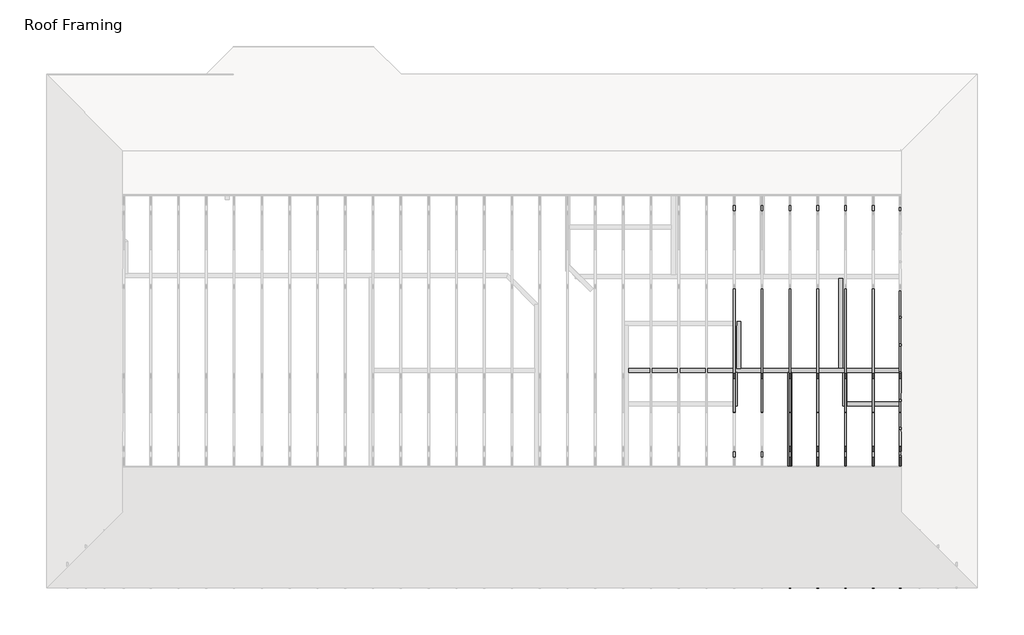
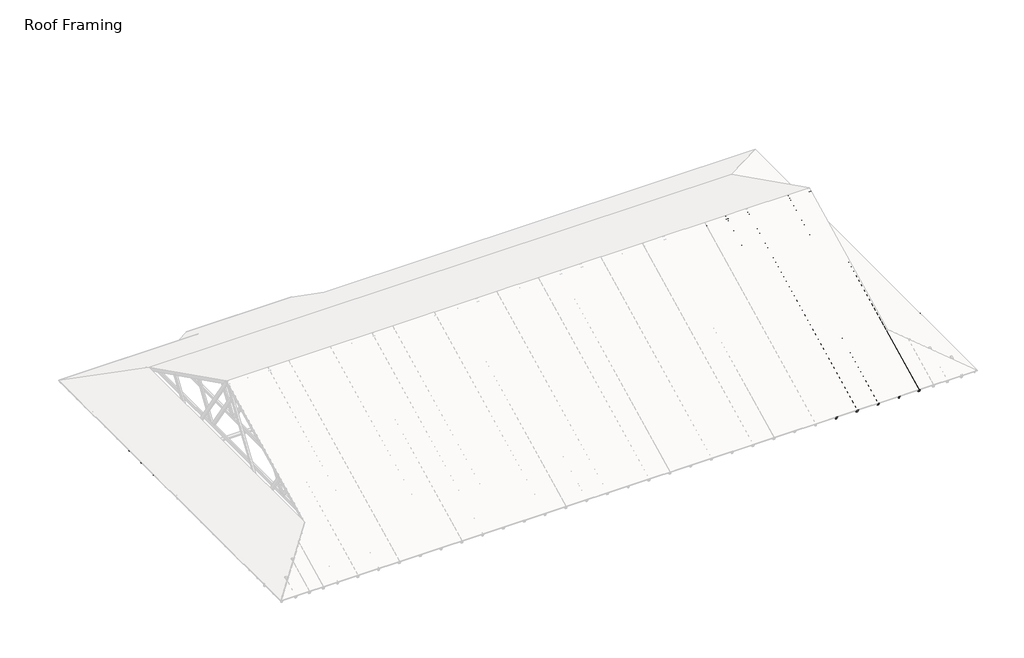
# One storey, part 4 of 7: 53 beams, 12 members.
"""IFC4 building model written with IfcOpenShell, lengths in millimetres."""

import ifcopenshell
import ifcopenshell.guid

model = None  # the IFC model being written
_history = None  # IfcOwnerHistory: only IFC2X3 demands one
_inside = {}  # id of a spatial element -> (the spatial element, [elements in it])
_under = {}  # id of a project, library or spatial element -> (it, [spatial elements below it])
_declared = {}  # id of a project -> (the project, [libraries it declares])
_typed = {}  # id of a type object -> (the type object, [elements of that type])
_made_of = {}  # id of a material, layer set ... -> (it, [elements and type objects made of it])


def new_model(schema):
    """Start an empty IFC model of exactly this schema.

    Asked for "IFC4X3", IfcOpenShell would pick the latest addendum, in which some entities
    have other attributes; the version numbers below select the first issue.
    IFC2X3 requires an IfcOwnerHistory on every rooted entity: one is made here for all.
    """
    global model, _history
    if schema == "IFC4X3":
        model = ifcopenshell.file(schema_version=(4, 3, 0, 0))
    else:
        model = ifcopenshell.file(schema=schema)
    _inside.clear()
    _under.clear()
    _declared.clear()
    _typed.clear()
    _made_of.clear()
    _history = None
    if model.schema == "IFC2X3":
        org = make("IfcOrganization", Name="unknown")
        user = make(
            "IfcPersonAndOrganization",
            ThePerson=make("IfcPerson", FamilyName="unknown"),
            TheOrganization=org,
        )
        app = make(
            "IfcApplication",
            ApplicationDeveloper=org,
            Version="unknown",
            ApplicationFullName="unknown",
            ApplicationIdentifier="unknown",
        )
        _history = make(
            "IfcOwnerHistory",
            OwningUser=user,
            OwningApplication=app,
            ChangeAction="ADDED",
            CreationDate=0,
        )
    return model


def make(cls, **values):
    """One entity of the class cls with the attributes given. An attribute that is None is left unset."""
    return model.create_entity(
        cls, **{name: value for name, value in values.items() if value is not None}
    )


def rooted(cls, **values):
    """An entity with a GlobalId (a new one), such as an element, a storey or a relation."""
    return make(cls, GlobalId=ifcopenshell.guid.new(), OwnerHistory=_history, **values)


def si_unit(unit_type, name, prefix=None):
    """IfcSIUnit, for example si_unit("LENGTHUNIT", "METRE", prefix="MILLI")."""
    return make("IfcSIUnit", UnitType=unit_type, Prefix=prefix, Name=name)


def assignment(units):
    """IfcUnitAssignment: the units of a project."""
    return None if units is None else make("IfcUnitAssignment", Units=units)


def point(xyz):
    """IfcCartesianPoint."""
    return None if xyz is None else make("IfcCartesianPoint", Coordinates=xyz)


def direction(xyz):
    """IfcDirection."""
    return None if xyz is None else make("IfcDirection", DirectionRatios=xyz)


def frame(location, z_axis=None, x_axis=None):
    """IfcAxis2Placement3D, a coordinate frame: its origin and axes. An axis left out is left unset."""
    return make(
        "IfcAxis2Placement3D",
        Location=point(location),
        Axis=direction(z_axis),
        RefDirection=direction(x_axis),
    )


def origin():
    """The frame at (0, 0, 0) with its axes left unset."""
    return frame((0.0, 0.0, 0.0))


def place(relative_to, where):
    """IfcLocalPlacement: puts the frame where relative to a parent placement (None: the world)."""
    return make(
        "IfcLocalPlacement", PlacementRelTo=relative_to, RelativePlacement=where
    )


def context(
    kind, dimensions, precision=None, world=None, true_north=None, identifier=None
):
    """IfcGeometricRepresentationContext, for example the 3D "Model" context."""
    return make(
        "IfcGeometricRepresentationContext",
        ContextIdentifier=identifier,
        ContextType=kind,
        CoordinateSpaceDimension=dimensions,
        Precision=precision,
        WorldCoordinateSystem=world,
        TrueNorth=true_north,
    )


def project(units=None, contexts=None):
    """IfcProject with its units and contexts."""
    return rooted(
        "IfcProject",
        Name="project",
        RepresentationContexts=contexts,
        UnitsInContext=assignment(units),
    )


def spatial(cls, under=None, at=None, **own):
    """A site, building, storey or space (cls), placed at a placement, below another one or the project."""
    s = rooted(cls, ObjectPlacement=at, **own)
    if under is not None:
        _under.setdefault(under.id(), (under, []))[1].append(s)
    return s


def polyline(points):
    """IfcPolyline through the points."""
    return make("IfcPolyline", Points=[point(p) for p in points])


def outline(outer, holes=None, kind="AREA"):
    """IfcArbitraryClosedProfileDef: a profile drawn as a closed curve; with holes, ...WithVoids."""
    if holes is None:
        return make("IfcArbitraryClosedProfileDef", ProfileType=kind, OuterCurve=outer)
    return make(
        "IfcArbitraryProfileDefWithVoids",
        ProfileType=kind,
        OuterCurve=outer,
        InnerCurves=holes,
    )


def extrude(swept, where, along, depth):
    """IfcExtrudedAreaSolid: the profile swept, set in the frame where, extruded along a direction by depth."""
    return make(
        "IfcExtrudedAreaSolid",
        SweptArea=swept,
        Position=where,
        ExtrudedDirection=direction(along),
        Depth=depth,
    )


def shape(context_of_items, identifier, shape_type, items):
    """IfcShapeRepresentation: the items that make up one representation, for example the "Body"."""
    return make(
        "IfcShapeRepresentation",
        ContextOfItems=context_of_items,
        RepresentationIdentifier=identifier,
        RepresentationType=shape_type,
        Items=items,
    )


def source(mapping_origin, context_of_items, identifier, shape_type, items):
    """IfcRepresentationMap: a shape defined once, which mapped items show again and again."""
    return make(
        "IfcRepresentationMap",
        MappingOrigin=mapping_origin,
        MappedRepresentation=shape(context_of_items, identifier, shape_type, items),
    )


def transform(
    local_origin,
    x_axis=None,
    y_axis=None,
    z_axis=None,
    scale=None,
    scale2=None,
    scale3=None,
    uniform=True,
):
    """IfcCartesianTransformationOperator3D, or its non-uniform kind. x_axis, y_axis, z_axis: its Axis1, 2, 3."""
    if uniform:
        return make(
            "IfcCartesianTransformationOperator3D",
            Axis1=direction(x_axis),
            Axis2=direction(y_axis),
            LocalOrigin=point(local_origin),
            Scale=scale,
            Axis3=direction(z_axis),
        )
    return make(
        "IfcCartesianTransformationOperator3DnonUniform",
        Axis1=direction(x_axis),
        Axis2=direction(y_axis),
        LocalOrigin=point(local_origin),
        Scale=scale,
        Axis3=direction(z_axis),
        Scale2=scale2,
        Scale3=scale3,
    )


def mapped(mapping_source, mapping_target):
    """IfcMappedItem: shows the shape of a source again, moved by a transform."""
    return make(
        "IfcMappedItem", MappingSource=mapping_source, MappingTarget=mapping_target
    )


def made_of(thing, what):
    """Note that an element or type object is made of a material, layer set ...; save() writes the relation."""
    if what is not None:
        _made_of.setdefault(what.id(), (what, []))[1].append(thing)
    return thing


def element(
    cls,
    number,
    at=None,
    inside=None,
    cuts=None,
    type_object=None,
    material=None,
    context=None,
    identifier="Body",
    shape_type=None,
    held_by="IfcProductDefinitionShape",
    body=None,
    shapes=None,
    **own,
):
    """One element of the class cls, such as IfcWall. Its Tag is "e" and its number.

    at: its placement. inside: the storey or other place that contains it. cuts: it is an
    opening in that element (IfcRelVoidsElement). A single representation is given by context,
    identifier, shape_type and body (its items); several are given by shapes. held_by: the class
    of the entity that holds the representations. save() writes the other relations.
    """
    e = rooted(cls, Tag="e%d" % number, ObjectPlacement=at, **own)
    if body is not None:
        shapes = [shape(context, identifier, shape_type, body)]
    if shapes is not None:
        e.Representation = make(held_by, Representations=shapes)
    if inside is not None:
        _inside.setdefault(inside.id(), (inside, []))[1].append(e)
    if cuts is not None:
        rooted(
            "IfcRelVoidsElement", RelatingBuildingElement=cuts, RelatedOpeningElement=e
        )
    if type_object is not None:
        _typed.setdefault(type_object.id(), (type_object, []))[1].append(e)
    return made_of(e, material)


def aggregate(whole, parts):
    """IfcRelAggregates: a whole, such as a stair, and the parts it consists of."""
    return rooted("IfcRelAggregates", RelatingObject=whole, RelatedObjects=parts)


def save(model, path):
    """Write the relations noted so far, then the file.

    IfcRelAggregates (storeys below a building ...), IfcRelContainedInSpatialStructure (elements
    in a storey), IfcRelDefinesByType, IfcRelAssociatesMaterial and IfcRelDeclares: one each for
    every whole, place, type object, material and project.
    """
    for whole, parts in _under.values():
        aggregate(whole, parts)
    for where, things in _inside.values():
        rooted(
            "IfcRelContainedInSpatialStructure",
            RelatedElements=things,
            RelatingStructure=where,
        )
    for kind, things in _typed.values():
        rooted("IfcRelDefinesByType", RelatedObjects=things, RelatingType=kind)
    for what, things in _made_of.values():
        rooted("IfcRelAssociatesMaterial", RelatedObjects=things, RelatingMaterial=what)
    for by, libraries in _declared.values():
        rooted("IfcRelDeclares", RelatingContext=by, RelatedDefinitions=libraries)
    model.write(path)


def dimension_lumber_c8f8d63a(model_context):
    return source(origin(), model_context, "Body", "SweptSolid", [
        extrude(outline(polyline([(5118.89375, 44.45), (5118.89375, -44.45), (-5118.89375, -44.45), (-5118.89375, 44.45), (5118.89375, 44.45)])), frame((0.0, 0.0, -19.05), z_axis=(0.0, 0.0, 1.0), x_axis=(1.0, 0.0, 0.0)), (0.0, 0.0, 1.0), 38.1),
    ])


def dimension_lumber_b8718559(model_context):
    return source(origin(), model_context, "Body", "SweptSolid", [
        extrude(outline(polyline([(987.425, 44.45), (987.425, -44.45), (-987.425, -44.45), (-987.425, 44.45), (987.425, 44.45)])), frame((0.0, 0.0, -19.05), z_axis=(0.0, 0.0, 1.0), x_axis=(1.0, 0.0, 0.0)), (0.0, 0.0, 1.0), 38.1),
    ])


def dimension_lumber_96205b60(model_context):
    return source(origin(), model_context, "Body", "SweptSolid", [
        extrude(outline(polyline([(3550.44375, 44.45), (3550.44375, -44.45), (-3550.44375, -44.45), (-3550.44375, 44.45), (3550.44375, 44.45)])), frame((0.0, 0.0, -19.05), z_axis=(0.0, 0.0, 1.0), x_axis=(1.0, 0.0, 0.0)), (0.0, 0.0, 1.0), 38.1),
    ])


def dimension_lumber_dd19c813(model_context):
    return source(origin(), model_context, "Body", "SweptSolid", [
        extrude(outline(polyline([(558.8, 44.45), (558.8, -44.45), (-469.9, -44.45), (-469.9, 44.45), (558.8, 44.45)])), frame((0.0, 0.0, -19.05), z_axis=(0.0, 0.0, 1.0), x_axis=(1.0, 0.0, 0.0)), (0.0, 0.0, 1.0), 38.1),
    ])


def dimension_lumber_d9c95be3(model_context):
    return source(origin(), model_context, "Body", "SweptSolid", [
        extrude(outline(polyline([(346.075, 44.45), (346.075, -44.45), (-384.175, -44.45), (-384.175, 44.45), (346.075, 44.45)])), frame((0.0, 0.0, -19.05), z_axis=(0.0, 0.0, 1.0), x_axis=(1.0, 0.0, 0.0)), (0.0, 0.0, 1.0), 38.1),
    ])


def dimension_lumber_c20748c8(model_context):
    return source(origin(), model_context, "Body", "SweptSolid", [
        extrude(outline(polyline([(1155.7, 44.45), (1155.7, -44.45), (-1155.7, -44.45), (-1155.7, 44.45), (1155.7, 44.45)])), frame((0.0, 0.0, -19.05), z_axis=(0.0, 0.0, 1.0), x_axis=(1.0, 0.0, 0.0)), (0.0, 0.0, 1.0), 38.1),
    ])


def dimension_lumber_348b767d(model_context):
    return source(origin(), model_context, "Body", "SweptSolid", [
        extrude(outline(polyline([(320.675, 44.45), (320.675, -44.45), (-409.575, -44.45), (-409.575, 44.45), (320.675, 44.45)])), frame((0.0, 0.0, -19.05), z_axis=(0.0, 0.0, 1.0), x_axis=(1.0, 0.0, 0.0)), (0.0, 0.0, 1.0), 38.1),
    ])


def dimension_lumber_22ea9708(model_context):
    return source(origin(), model_context, "Body", "SweptSolid", [
        extrude(outline(polyline([(2035.175, 44.45), (2035.175, -44.45), (-2035.175, -44.45), (-2035.175, 44.45), (2035.175, 44.45)])), frame((0.0, 0.0, -19.05), z_axis=(0.0, 0.0, 1.0), x_axis=(1.0, 0.0, 0.0)), (0.0, 0.0, 1.0), 38.1),
    ])


def dimension_lumber_74193215(model_context):
    return source(origin(), model_context, "Body", "SweptSolid", [
        extrude(outline(polyline([(409.575, 44.45), (409.575, -44.45), (-320.675, -44.45), (-320.675, 44.45), (409.575, 44.45)])), frame((0.0, 0.0, -19.05), z_axis=(0.0, 0.0, 1.0), x_axis=(1.0, 0.0, 0.0)), (0.0, 0.0, 1.0), 38.1),
    ])


def dimension_lumber_7189ff9c(model_context):
    return source(origin(), model_context, "Body", "SweptSolid", [
        extrude(outline(polyline([(1146.96875, 44.45), (1146.96875, -44.45), (-1164.43125, -44.45), (-1164.43125, 44.45), (1146.96875, 44.45)])), frame((0.0, 0.0, -19.05), z_axis=(0.0, 0.0, 1.0), x_axis=(1.0, 0.0, 0.0)), (0.0, 0.0, 1.0), 38.1),
    ])


def dimension_lumber_f425b765(model_context):
    return source(origin(), model_context, "Body", "SweptSolid", [
        extrude(outline(polyline([(292.0, 44.45), (292.0, -44.45), (-165.0, -44.45), (-165.0, 44.45), (292.0, 44.45)])), frame((0.0, 0.0, -19.05), z_axis=(0.0, 0.0, 1.0), x_axis=(1.0, 0.0, 0.0)), (0.0, 0.0, 1.0), 38.1),
    ])


def dimension_lumber_supporting_bottom_plate_e3733361(model_context):
    return source(origin(), model_context, "Body", "SweptSolid", [
        extrude(outline(polyline([(328.9051334, 44.45), (328.9051334, -44.45), (-328.9051334, -44.45), (-328.9051334, 44.45), (328.9051334, 44.45)])), frame((0.0, 0.0, -19.05), z_axis=(0.0, 0.0, 1.0), x_axis=(1.0, 0.0, 0.0)), (0.0, 0.0, 1.0), 38.1),
    ])


def dimension_lumber_supporting_bottom_plate_47a8c852(model_context):
    return source(origin(), model_context, "Body", "SweptSolid", [
        extrude(outline(polyline([(292.0, 44.45), (292.0, -44.45), (-203.1, -44.45), (-203.1, 44.45), (292.0, 44.45)])), frame((0.0, 0.0, -19.05), z_axis=(0.0, 0.0, 1.0), x_axis=(1.0, 0.0, 0.0)), (0.0, 0.0, 1.0), 38.1),
    ])


model = new_model("IFC4")

# Units and contexts
model_context = context("Model", 3, world=origin())
ifc_project = project(units=[si_unit("LENGTHUNIT", "METRE", prefix="MILLI")], contexts=[model_context])

# Site, building, storey
site = spatial("IfcSite", under=ifc_project)
building = spatial("IfcBuilding", under=site)
storey = spatial("IfcBuildingStorey", under=building, Name="Roof Framing", Elevation=2768.6)

# Beams
placement = place(None, origin())
element("IfcBeam", 1, ObjectType="Dimension Lumber : Roof Lumbers", at=placement, inside=storey, context=model_context, shape_type="SweptSolid", body=[
    extrude(outline(polyline([(0.0, -38.1), (0.0, 0.0), (1874.2721787, 0.0), (1874.2721787, -38.1), (0.0, -38.1)])), frame((13672.6274862, -3444.5040947, 2554.840297), z_axis=(0.44721359549993345, 0.0, 0.8944271909999282), x_axis=(-0.8944271909999282, 0.0, 0.44721359549993345)), (0.0, 0.0, 1.0), 88.9),
    extrude(outline(polyline([(2554.840297, 13672.6274862), (2558.1548743, 13674.2847749), (2653.4048743, 13674.2847749), (3472.5548743, 12035.9847749), (3393.040297, 11996.2274862), (2554.840297, 13672.6274862)])), frame((0.0, -3444.5040947, 0.0), z_axis=(0.0, 1.0, 0.0), x_axis=(0.0, 0.0, 1.0)), (0.0, 0.0, 1.0), 38.1),
    extrude(outline(polyline([(2554.840297, 13672.6274862), (2558.1548743, 13674.2847749), (2653.4048743, 13674.2847749), (3472.5548743, 12035.9847749), (3373.1616527, 12035.9847749), (2554.840297, 13672.6274862)])), frame((0.0, -3444.5040947, 0.0), z_axis=(0.0, 1.0, 0.0), x_axis=(0.0, 0.0, 1.0)), (0.0, 0.0, 1.0), 38.1),
])
element("IfcBeam", 2, ObjectType="Dimension Lumber : Roof Lumbers", at=placement, inside=storey, context=model_context, shape_type="SweptSolid", body=[
    extrude(outline(polyline([(0.0, -38.1), (0.0, 0.0), (1874.2721787, 0.0), (1874.2721787, -38.1), (0.0, -38.1)])), frame((13672.6274862, -2834.9040947, 2554.840297), z_axis=(0.44721359549993345, 0.0, 0.8944271909999282), x_axis=(-0.8944271909999282, 0.0, 0.44721359549993345)), (0.0, 0.0, 1.0), 88.9),
    extrude(outline(polyline([(2554.840297, 13672.6274862), (2558.1548743, 13674.2847749), (2653.4048743, 13674.2847749), (3472.5548743, 12035.9847749), (3393.040297, 11996.2274862), (2554.840297, 13672.6274862)])), frame((0.0, -2834.9040947, 0.0), z_axis=(0.0, 1.0, 0.0), x_axis=(0.0, 0.0, 1.0)), (0.0, 0.0, 1.0), 38.1),
    extrude(outline(polyline([(2554.840297, 13672.6274862), (2558.1548743, 13674.2847749), (2653.4048743, 13674.2847749), (3472.5548743, 12035.9847749), (3373.1616527, 12035.9847749), (2554.840297, 13672.6274862)])), frame((0.0, -2834.9040947, 0.0), z_axis=(0.0, 1.0, 0.0), x_axis=(0.0, 0.0, 1.0)), (0.0, 0.0, 1.0), 38.1),
])
element("IfcBeam", 3, ObjectType="Dimension Lumber : Roof Lumbers", at=placement, inside=storey, context=model_context, shape_type="SweptSolid", body=[
    extrude(outline(polyline([(0.0, -38.1), (0.0, 0.0), (1874.2721787, 0.0), (1874.2721787, -38.1), (0.0, -38.1)])), frame((13672.6274862, -2225.3040947, 2554.840297), z_axis=(0.44721359549993345, 0.0, 0.8944271909999282), x_axis=(-0.8944271909999282, 0.0, 0.44721359549993345)), (0.0, 0.0, 1.0), 88.9),
    extrude(outline(polyline([(2554.840297, 13672.6274862), (2558.1548743, 13674.2847749), (2653.4048743, 13674.2847749), (3472.5548743, 12035.9847749), (3393.040297, 11996.2274862), (2554.840297, 13672.6274862)])), frame((0.0, -2225.3040947, 0.0), z_axis=(0.0, 1.0, 0.0), x_axis=(0.0, 0.0, 1.0)), (0.0, 0.0, 1.0), 38.1),
    extrude(outline(polyline([(2554.840297, 13672.6274862), (2558.1548743, 13674.2847749), (2653.4048743, 13674.2847749), (3472.5548743, 12035.9847749), (3373.1616527, 12035.9847749), (2554.840297, 13672.6274862)])), frame((0.0, -2225.3040947, 0.0), z_axis=(0.0, 1.0, 0.0), x_axis=(0.0, 0.0, 1.0)), (0.0, 0.0, 1.0), 38.1),
])
element("IfcBeam", 4, ObjectType="Dimension Lumber : Roof Lumbers", at=placement, inside=storey, context=model_context, shape_type="SweptSolid", body=[
    extrude(outline(polyline([(0.0, -38.1), (0.0, 0.0), (1874.2721787, 0.0), (1874.2721787, -38.1), (0.0, -38.1)])), frame((13672.6274862, -1006.1040947, 2554.840297), z_axis=(0.44721359549993367, 0.0, 0.8944271909999281), x_axis=(-0.8944271909999281, 0.0, 0.44721359549993367)), (0.0, 0.0, 1.0), 88.9),
    extrude(outline(polyline([(2554.840297, 13672.6274862), (2558.1548743, 13674.2847749), (2653.4048743, 13674.2847749), (3472.5548743, 12035.9847749), (3393.040297, 11996.2274862), (2554.840297, 13672.6274862)])), frame((0.0, -1006.1040947, 0.0), z_axis=(0.0, 1.0, 0.0), x_axis=(0.0, 0.0, 1.0)), (0.0, 0.0, 1.0), 38.1),
    extrude(outline(polyline([(2554.840297, 13672.6274862), (2558.1548743, 13674.2847749), (2653.4048743, 13674.2847749), (3472.5548743, 12035.9847749), (3373.1616527, 12035.9847749), (2554.840297, 13672.6274862)])), frame((0.0, -1006.1040947, 0.0), z_axis=(0.0, 1.0, 0.0), x_axis=(0.0, 0.0, 1.0)), (0.0, 0.0, 1.0), 38.1),
])
element("IfcBeam", 5, ObjectType="Dimension Lumber : Roof Lumbers", at=placement, inside=storey, context=model_context, shape_type="SweptSolid", body=[
    extrude(outline(polyline([(0.0, -38.1), (0.0, 0.0), (1874.2721787, 0.0), (1874.2721787, -38.1), (0.0, -38.1)])), frame((13672.6274862, -396.5040947, 2554.840297), z_axis=(0.44721359549993345, 0.0, 0.8944271909999282), x_axis=(-0.8944271909999282, 0.0, 0.44721359549993345)), (0.0, 0.0, 1.0), 88.9),
    extrude(outline(polyline([(2554.840297, 13672.6274862), (2558.1548743, 13674.2847749), (2653.4048743, 13674.2847749), (3472.5548743, 12035.9847749), (3393.040297, 11996.2274862), (2554.840297, 13672.6274862)])), frame((0.0, -396.5040947, 0.0), z_axis=(0.0, 1.0, 0.0), x_axis=(0.0, 0.0, 1.0)), (0.0, 0.0, 1.0), 38.1),
    extrude(outline(polyline([(2554.840297, 13672.6274862), (2558.1548743, 13674.2847749), (2653.4048743, 13674.2847749), (3472.5548743, 12035.9847749), (3373.1616527, 12035.9847749), (2554.840297, 13672.6274862)])), frame((0.0, -396.5040947, 0.0), z_axis=(0.0, 1.0, 0.0), x_axis=(0.0, 0.0, 1.0)), (0.0, 0.0, 1.0), 38.1),
])
element("IfcBeam", 6, ObjectType="Dimension Lumber : Roof Lumbers", at=placement, inside=storey, context=model_context, shape_type="SweptSolid", body=[
    extrude(outline(polyline([(12035.9847749, -3406.4040947), (13244.0722749, -3406.4040947), (13244.0722749, -3444.5040947), (12035.9847749, -3444.5040947), (12035.9847749, -3406.4040947)])), frame((0.0, 0.0, 2768.6), z_axis=(0.0, 0.0, 1.0), x_axis=(1.0, 0.0, 0.0)), (0.0, 0.0, 1.0), 88.9),
    extrude(outline(polyline([(2768.6, 12035.9847749), (2768.6, 13244.0722749), (2769.1179027, 13244.0722749), (2857.5, 13067.3080803), (2857.5, 12035.9847749), (2768.6, 12035.9847749)])), frame((0.0, -3444.5040947, 0.0), z_axis=(0.0, 1.0, 0.0), x_axis=(0.0, 0.0, 1.0)), (0.0, 0.0, 1.0), 38.1),
])
element("IfcBeam", 7, ObjectType="Dimension Lumber : Roof Lumbers", at=placement, inside=storey, context=model_context, shape_type="SweptSolid", body=[
    extrude(outline(polyline([(12035.9847749, -2796.8040947), (13244.0722749, -2796.8040947), (13244.0722749, -2834.9040947), (12035.9847749, -2834.9040947), (12035.9847749, -2796.8040947)])), frame((0.0, 0.0, 2768.6), z_axis=(0.0, 0.0, 1.0), x_axis=(1.0, 0.0, 0.0)), (0.0, 0.0, 1.0), 88.9),
    extrude(outline(polyline([(2768.6, 12035.9847749), (2768.6, 13244.0722749), (2769.1179027, 13244.0722749), (2857.5, 13067.3080803), (2857.5, 12035.9847749), (2768.6, 12035.9847749)])), frame((0.0, -2834.9040947, 0.0), z_axis=(0.0, 1.0, 0.0), x_axis=(0.0, 0.0, 1.0)), (0.0, 0.0, 1.0), 38.1),
])
element("IfcBeam", 8, ObjectType="Dimension Lumber : Roof Lumbers", at=placement, inside=storey, context=model_context, shape_type="SweptSolid", body=[
    extrude(outline(polyline([(12035.9847749, -2187.2040947), (13244.0722749, -2187.2040947), (13244.0722749, -2225.3040947), (12035.9847749, -2225.3040947), (12035.9847749, -2187.2040947)])), frame((0.0, 0.0, 2768.6), z_axis=(0.0, 0.0, 1.0), x_axis=(1.0, 0.0, 0.0)), (0.0, 0.0, 1.0), 88.9),
    extrude(outline(polyline([(2768.6, 12035.9847749), (2768.6, 13244.0722749), (2769.1179027, 13244.0722749), (2857.5, 13067.3080803), (2857.5, 12035.9847749), (2768.6, 12035.9847749)])), frame((0.0, -2225.3040947, 0.0), z_axis=(0.0, 1.0, 0.0), x_axis=(0.0, 0.0, 1.0)), (0.0, 0.0, 1.0), 38.1),
])
element("IfcBeam", 9, ObjectType="Dimension Lumber : Roof Lumbers", at=placement, inside=storey, context=model_context, shape_type="SweptSolid", body=[
    extrude(outline(polyline([(12035.9847749, -1577.6040947), (13244.0722749, -1577.6040947), (13244.0722749, -1615.7040947), (12035.9847749, -1615.7040947), (12035.9847749, -1577.6040947)])), frame((0.0, 0.0, 2768.6), z_axis=(0.0, 0.0, 1.0), x_axis=(1.0, 0.0, 0.0)), (0.0, 0.0, 1.0), 88.9),
    extrude(outline(polyline([(2768.6, 12035.9847749), (2768.6, 13244.0722749), (2769.1179027, 13244.0722749), (2857.5, 13067.3080803), (2857.5, 12035.9847749), (2768.6, 12035.9847749)])), frame((0.0, -1615.7040947, 0.0), z_axis=(0.0, 1.0, 0.0), x_axis=(0.0, 0.0, 1.0)), (0.0, 0.0, 1.0), 38.1),
])
element("IfcBeam", 10, ObjectType="Dimension Lumber : Roof Lumbers", at=placement, inside=storey, context=model_context, shape_type="SweptSolid", body=[
    extrude(outline(polyline([(12035.9847749, -968.0040947), (13244.0722749, -968.0040947), (13244.0722749, -1006.1040947), (12035.9847749, -1006.1040947), (12035.9847749, -968.0040947)])), frame((0.0, 0.0, 2768.6), z_axis=(0.0, 0.0, 1.0), x_axis=(1.0, 0.0, 0.0)), (0.0, 0.0, 1.0), 88.9),
    extrude(outline(polyline([(2768.6, 12035.9847749), (2768.6, 13244.0722749), (2769.1179027, 13244.0722749), (2857.5, 13067.3080803), (2857.5, 12035.9847749), (2768.6, 12035.9847749)])), frame((0.0, -1006.1040947, 0.0), z_axis=(0.0, 1.0, 0.0), x_axis=(0.0, 0.0, 1.0)), (0.0, 0.0, 1.0), 38.1),
])
element("IfcBeam", 11, ObjectType="Dimension Lumber : Roof Lumbers", at=placement, inside=storey, context=model_context, shape_type="SweptSolid", body=[
    extrude(outline(polyline([(12035.9847749, -358.4040947), (13244.0722749, -358.4040947), (13244.0722749, -396.5040947), (12035.9847749, -396.5040947), (12035.9847749, -358.4040947)])), frame((0.0, 0.0, 2768.6), z_axis=(0.0, 0.0, 1.0), x_axis=(1.0, 0.0, 0.0)), (0.0, 0.0, 1.0), 88.9),
    extrude(outline(polyline([(2768.6, 12035.9847749), (2768.6, 13244.0722749), (2769.1179027, 13244.0722749), (2857.5, 13067.3080803), (2857.5, 12035.9847749), (2768.6, 12035.9847749)])), frame((0.0, -396.5040947, 0.0), z_axis=(0.0, 1.0, 0.0), x_axis=(0.0, 0.0, 1.0)), (0.0, 0.0, 1.0), 38.1),
])
element("IfcBeam", 12, ObjectType="Dimension Lumber : Roof Lumbers", at=placement, inside=storey, context=model_context, shape_type="SweptSolid", body=[
    extrude(outline(polyline([(0.0, -38.1), (0.0, 0.0), (1874.2721787, 0.0), (1874.2721787, -38.1), (0.0, -38.1)])), frame((13672.6274862, -1615.7040947, 2554.840297), z_axis=(0.44721359549993367, 0.0, 0.8944271909999281), x_axis=(-0.8944271909999281, 0.0, 0.44721359549993367)), (0.0, 0.0, 1.0), 88.9),
    extrude(outline(polyline([(2554.840297, 13672.6274862), (2558.1548743, 13674.2847749), (2653.4048743, 13674.2847749), (3472.5548743, 12035.9847749), (3393.040297, 11996.2274862), (2554.840297, 13672.6274862)])), frame((0.0, -1615.7040947, 0.0), z_axis=(0.0, 1.0, 0.0), x_axis=(0.0, 0.0, 1.0)), (0.0, 0.0, 1.0), 38.1),
    extrude(outline(polyline([(2554.840297, 13672.6274862), (2558.1548743, 13674.2847749), (2653.4048743, 13674.2847749), (3472.5548743, 12035.9847749), (3373.1616527, 12035.9847749), (2554.840297, 13672.6274862)])), frame((0.0, -1615.7040947, 0.0), z_axis=(0.0, 1.0, 0.0), x_axis=(0.0, 0.0, 1.0)), (0.0, 0.0, 1.0), 38.1),
])
element("IfcBeam", 13, ObjectType="Dimension Lumber : Roof Lumbers", at=placement, inside=storey, context=model_context, shape_type="SweptSolid", body=[
    extrude(outline(polyline([(13255.1847749, -5901.9540947), (13255.1847749, 4537.4459053), (13293.2847749, 4537.4459053), (13293.2847749, -5901.9540947), (13255.1847749, -5901.9540947)])), frame((0.0, 0.0, 2564.60625), z_axis=(0.0, 0.0, 1.0), x_axis=(1.0, 0.0, 0.0)), (0.0, 0.0, 1.0), 88.9),
])
dimension_lumber_shape = dimension_lumber_c8f8d63a(model_context)
element("IfcBeam", 14, ObjectType="Dimension Lumber : Top Supporting Lumbers", at=placement, inside=storey, context=model_context, shape_type="MappedRepresentation", body=[
    mapped(dimension_lumber_shape, transform((13199.6222749, -630.6603447, 2711.45), x_axis=(0.0, -1.0, 0.0), y_axis=(1.0, 0.0, 0.0), z_axis=(0.0, 0.0, 1.0))),
])
dimension_lumber_2_shape = dimension_lumber_b8718559(model_context)
element("IfcBeam", 15, ObjectType="Dimension Lumber : Top Supporting Lumbers", at=placement, inside=storey, context=model_context, shape_type="MappedRepresentation", body=[
    mapped(dimension_lumber_2_shape, transform((10715.1847749, -513.9790947, 2711.45), x_axis=(0.0, -1.0, 0.0), y_axis=(1.0, 0.0, 0.0), z_axis=(0.0, 0.0, 1.0))),
])
dimension_lumber_3_shape = dimension_lumber_96205b60(model_context)
element("IfcBeam", 16, ObjectType="Dimension Lumber : Top Supporting Lumbers", at=placement, inside=storey, context=model_context, shape_type="MappedRepresentation", body=[
    mapped(dimension_lumber_3_shape, transform((9604.7285249, -1545.8540947, 2711.45), x_axis=(-1.0, 0.0, 0.0), y_axis=(0.0, -1.0, 0.0), z_axis=(0.0, 0.0, 1.0))),
])
dimension_lumber_4_shape = dimension_lumber_dd19c813(model_context)
element("IfcBeam", 17, ObjectType="Dimension Lumber : Top Supporting Lumbers", at=placement, inside=storey, context=model_context, shape_type="MappedRepresentation", body=[
    mapped(dimension_lumber_4_shape, transform((8479.9847749, -1031.5040947, 2711.45), x_axis=(0.0, 1.0, 0.0), y_axis=(-1.0, 0.0, 0.0), z_axis=(0.0, 0.0, 1.0))),
])
dimension_lumber_5_shape = dimension_lumber_d9c95be3(model_context)
element("IfcBeam", 18, ObjectType="Dimension Lumber : Top Supporting Lumbers", at=placement, inside=storey, context=model_context, shape_type="MappedRepresentation", body=[
    mapped(dimension_lumber_5_shape, transform((8397.4347755, -1936.3790947, 2711.45), x_axis=(0.0, 1.0, 0.0), y_axis=(-1.0, 0.0, 0.0), z_axis=(0.0, 0.0, 1.0))),
])
dimension_lumber_6_shape = dimension_lumber_c20748c8(model_context)
element("IfcBeam", 19, ObjectType="Dimension Lumber : Top Supporting Lumbers", at=placement, inside=storey, context=model_context, shape_type="MappedRepresentation", body=[
    mapped(dimension_lumber_6_shape, transform((11999.4722749, -2276.1040947, 2711.45), x_axis=(1.0, 0.0, 0.0), y_axis=(0.0, 1.0, 0.0), z_axis=(0.0, 0.0, 1.0))),
])
dimension_lumber_7_shape = dimension_lumber_348b767d(model_context)
element("IfcBeam", 20, ObjectType="Dimension Lumber : Top Supporting Lumbers", at=placement, inside=storey, context=model_context, shape_type="MappedRepresentation", body=[
    mapped(dimension_lumber_7_shape, transform((10799.3222749, -1910.9790947, 2711.45), x_axis=(0.0, 1.0, 0.0), y_axis=(-1.0, 0.0, 0.0), z_axis=(0.0, 0.0, 1.0))),
])
dimension_lumber_8_shape = dimension_lumber_22ea9708(model_context)
element("IfcBeam", 21, ObjectType="Dimension Lumber : Top Supporting Lumbers", at=placement, inside=storey, context=model_context, shape_type="MappedRepresentation", body=[
    mapped(dimension_lumber_8_shape, transform((9597.5847749, -3625.4790947, 2711.45), x_axis=(0.0, -1.0, 0.0), y_axis=(1.0, 0.0, 0.0), z_axis=(0.0, 0.0, 1.0))),
])
element("IfcBeam", 22, ObjectType="Dimension Lumber : Top Supporting Lumbers", at=placement, inside=storey, context=model_context, shape_type="MappedRepresentation", body=[
    mapped(dimension_lumber_2_shape, transform((10715.1847749, -513.9790947, 2749.55), x_axis=(0.0, -1.0, 0.0), y_axis=(1.0, 0.0, 0.0), z_axis=(0.0, 0.0, 1.0))),
])
element("IfcBeam", 23, ObjectType="Dimension Lumber : Top Supporting Lumbers", at=placement, inside=storey, context=model_context, shape_type="MappedRepresentation", body=[
    mapped(dimension_lumber_3_shape, transform((9604.7285249, -1545.8540947, 2749.55), x_axis=(-1.0, 0.0, 0.0), y_axis=(0.0, -1.0, 0.0), z_axis=(0.0, 0.0, 1.0))),
])
element("IfcBeam", 24, ObjectType="Dimension Lumber : Top Supporting Lumbers", at=placement, inside=storey, context=model_context, shape_type="MappedRepresentation", body=[
    mapped(dimension_lumber_4_shape, transform((8479.9847749, -1031.5040947, 2749.55), x_axis=(0.0, 1.0, 0.0), y_axis=(-1.0, 0.0, 0.0), z_axis=(0.0, 0.0, 1.0))),
])
dimension_lumber_9_shape = dimension_lumber_74193215(model_context)
element("IfcBeam", 25, ObjectType="Dimension Lumber : Top Supporting Lumbers", at=placement, inside=storey, context=model_context, shape_type="MappedRepresentation", body=[
    mapped(dimension_lumber_9_shape, transform((8397.4347755, -1910.9790947, 2749.55), x_axis=(0.0, -1.0, 0.0), y_axis=(1.0, 0.0, 0.0), z_axis=(0.0, 0.0, 1.0))),
])
element("IfcBeam", 26, ObjectType="Dimension Lumber : Top Supporting Lumbers", at=placement, inside=storey, context=model_context, shape_type="MappedRepresentation", body=[
    mapped(dimension_lumber_8_shape, transform((9597.5847749, -3625.4790947, 2749.55), x_axis=(0.0, -1.0, 0.0), y_axis=(1.0, 0.0, 0.0), z_axis=(0.0, 0.0, 1.0))),
])
element("IfcBeam", 27, ObjectType="Dimension Lumber : Top Supporting Lumbers", at=placement, inside=storey, context=model_context, shape_type="MappedRepresentation", body=[
    mapped(dimension_lumber_9_shape, transform((10799.3222749, -1910.9790947, 2749.55), x_axis=(0.0, -1.0, 0.0), y_axis=(1.0, 0.0, 0.0), z_axis=(0.0, 0.0, 1.0))),
])
dimension_lumber_10_shape = dimension_lumber_7189ff9c(model_context)
element("IfcBeam", 28, ObjectType="Dimension Lumber : Top Supporting Lumbers", at=placement, inside=storey, context=model_context, shape_type="MappedRepresentation", body=[
    mapped(dimension_lumber_10_shape, transform((12008.2035249, -2276.1040947, 2749.55), x_axis=(1.0, 0.0, 0.0), y_axis=(0.0, 1.0, 0.0), z_axis=(0.0, 0.0, 1.0))),
])
dimension_lumber_11_shape = dimension_lumber_f425b765(model_context)
element("IfcBeam", 29, ObjectType="Dimension Lumber : Top Supporting Lumbers", at=placement, inside=storey, context=model_context, shape_type="MappedRepresentation", body=[
    mapped(dimension_lumber_11_shape, transform((12452.9120082, -1298.3040947, 2711.45), x_axis=(0.0, 1.0, 0.0), y_axis=(-1.0, 0.0, 0.0), z_axis=(0.0, 0.0, 1.0))),
])
dimension_lumber_supporting_bottom_plate_shape = dimension_lumber_supporting_bottom_plate_e3733361(model_context)
element("IfcBeam", 30, ObjectType="Dimension Lumber : Top Supporting Lumbers", at=placement, inside=storey, context=model_context, shape_type="MappedRepresentation", body=[
    mapped(dimension_lumber_supporting_bottom_plate_shape, transform((12826.2671415, -1050.7540947, 2711.45), x_axis=(1.0, 0.0, 0.0), y_axis=(0.0, 1.0, 0.0), z_axis=(0.0, 0.0, 1.0))),
])
element("IfcBeam", 31, ObjectType="Dimension Lumber : Top Supporting Lumbers", at=placement, inside=storey, context=model_context, shape_type="MappedRepresentation", body=[
    mapped(dimension_lumber_supporting_bottom_plate_shape, transform((12826.2671415, -1050.7540947, 2749.55), x_axis=(1.0, 0.0, 0.0), y_axis=(0.0, 1.0, 0.0), z_axis=(0.0, 0.0, 1.0))),
])
dimension_lumber_supporting_bottom_plate_2_shape = dimension_lumber_supporting_bottom_plate_47a8c852(model_context)
element("IfcBeam", 32, ObjectType="Dimension Lumber : Top Supporting Lumbers", at=placement, inside=storey, context=model_context, shape_type="MappedRepresentation", body=[
    mapped(dimension_lumber_supporting_bottom_plate_2_shape, transform((12452.9120082, -1298.3040947, 2749.55), x_axis=(0.0, 1.0, 0.0), y_axis=(-1.0, 0.0, 0.0), z_axis=(0.0, 0.0, 1.0))),
])
element("IfcBeam", 33, ObjectType="Dimension Lumber : 2x4 Blocking", at=placement, inside=storey, context=model_context, shape_type="SweptSolid", body=[
    extrude(outline(polyline([(13674.2847749, -3444.5040947), (13293.2847749, -3444.5040947), (13293.2847749, -3406.4040947), (13674.2847749, -3406.4040947), (13674.2847749, -3444.5040947)])), frame((0.0, 0.0, 2564.60625), z_axis=(0.0, 0.0, 1.0), x_axis=(1.0, 0.0, 0.0)), (0.0, 0.0, 1.0), 88.9),
    extrude(outline(polyline([(2653.50625, 13475.2955803), (2653.50625, 13293.2847749), (2564.60625, 13293.2847749), (2564.60625, 13653.0955803), (2653.50625, 13475.2955803)])), frame((0.0, -3444.5040947, 0.0), z_axis=(0.0, 1.0, 0.0), x_axis=(0.0, 0.0, 1.0)), (0.0, 0.0, 1.0), 38.1),
])
element("IfcBeam", 34, ObjectType="Dimension Lumber : 2x4 Blocking", at=placement, inside=storey, context=model_context, shape_type="SweptSolid", body=[
    extrude(outline(polyline([(13674.2847749, -2834.9040947), (13293.2847749, -2834.9040947), (13293.2847749, -2796.8040947), (13674.2847749, -2796.8040947), (13674.2847749, -2834.9040947)])), frame((0.0, 0.0, 2564.60625), z_axis=(0.0, 0.0, 1.0), x_axis=(1.0, 0.0, 0.0)), (0.0, 0.0, 1.0), 88.9),
    extrude(outline(polyline([(2653.50625, 13475.2955803), (2653.50625, 13293.2847749), (2564.60625, 13293.2847749), (2564.60625, 13653.0955803), (2653.50625, 13475.2955803)])), frame((0.0, -2834.9040947, 0.0), z_axis=(0.0, 1.0, 0.0), x_axis=(0.0, 0.0, 1.0)), (0.0, 0.0, 1.0), 38.1),
])
element("IfcBeam", 35, ObjectType="Dimension Lumber : 2x4 Blocking", at=placement, inside=storey, context=model_context, shape_type="SweptSolid", body=[
    extrude(outline(polyline([(13674.2847749, -2225.3040947), (13293.2847749, -2225.3040947), (13293.2847749, -2187.2040947), (13674.2847749, -2187.2040947), (13674.2847749, -2225.3040947)])), frame((0.0, 0.0, 2564.60625), z_axis=(0.0, 0.0, 1.0), x_axis=(1.0, 0.0, 0.0)), (0.0, 0.0, 1.0), 88.9),
    extrude(outline(polyline([(2653.50625, 13475.2955803), (2653.50625, 13293.2847749), (2564.60625, 13293.2847749), (2564.60625, 13653.0955803), (2653.50625, 13475.2955803)])), frame((0.0, -2225.3040947, 0.0), z_axis=(0.0, 1.0, 0.0), x_axis=(0.0, 0.0, 1.0)), (0.0, 0.0, 1.0), 38.1),
])
element("IfcBeam", 36, ObjectType="Dimension Lumber : 2x4 Blocking", at=placement, inside=storey, context=model_context, shape_type="SweptSolid", body=[
    extrude(outline(polyline([(13674.2847749, -1615.7040947), (13293.2847749, -1615.7040947), (13293.2847749, -1577.6040947), (13674.2847749, -1577.6040947), (13674.2847749, -1615.7040947)])), frame((0.0, 0.0, 2564.60625), z_axis=(0.0, 0.0, 1.0), x_axis=(1.0, 0.0, 0.0)), (0.0, 0.0, 1.0), 88.9),
    extrude(outline(polyline([(2653.50625, 13475.2955803), (2653.50625, 13293.2847749), (2564.60625, 13293.2847749), (2564.60625, 13653.0955803), (2653.50625, 13475.2955803)])), frame((0.0, -1615.7040947, 0.0), z_axis=(0.0, 1.0, 0.0), x_axis=(0.0, 0.0, 1.0)), (0.0, 0.0, 1.0), 38.1),
])
element("IfcBeam", 37, ObjectType="Dimension Lumber : 2x4 Blocking", at=placement, inside=storey, context=model_context, shape_type="SweptSolid", body=[
    extrude(outline(polyline([(13674.2847749, -1006.1040947), (13293.2847749, -1006.1040947), (13293.2847749, -968.0040947), (13674.2847749, -968.0040947), (13674.2847749, -1006.1040947)])), frame((0.0, 0.0, 2564.60625), z_axis=(0.0, 0.0, 1.0), x_axis=(1.0, 0.0, 0.0)), (0.0, 0.0, 1.0), 88.9),
    extrude(outline(polyline([(2653.50625, 13475.2955803), (2653.50625, 13293.2847749), (2564.60625, 13293.2847749), (2564.60625, 13653.0955803), (2653.50625, 13475.2955803)])), frame((0.0, -1006.1040947, 0.0), z_axis=(0.0, 1.0, 0.0), x_axis=(0.0, 0.0, 1.0)), (0.0, 0.0, 1.0), 38.1),
])
element("IfcBeam", 38, ObjectType="Dimension Lumber : 2x4 Blocking", at=placement, inside=storey, context=model_context, shape_type="SweptSolid", body=[
    extrude(outline(polyline([(13674.2847749, -396.5040947), (13293.2847749, -396.5040947), (13293.2847749, -358.4040947), (13674.2847749, -358.4040947), (13674.2847749, -396.5040947)])), frame((0.0, 0.0, 2564.60625), z_axis=(0.0, 0.0, 1.0), x_axis=(1.0, 0.0, 0.0)), (0.0, 0.0, 1.0), 88.9),
    extrude(outline(polyline([(2653.50625, 13475.2955803), (2653.50625, 13293.2847749), (2564.60625, 13293.2847749), (2564.60625, 13653.0955803), (2653.50625, 13475.2955803)])), frame((0.0, -396.5040947, 0.0), z_axis=(0.0, 1.0, 0.0), x_axis=(0.0, 0.0, 1.0)), (0.0, 0.0, 1.0), 38.1),
])
element("IfcBeam", 39, ObjectType="Dimension Lumber : 2x4 Blocking", at=placement, inside=storey, context=model_context, shape_type="SweptSolid", body=[
    extrude(outline(polyline([(-6671.1152251, 213.0959053), (-6671.1152251, 251.1959053), (-6290.1152251, 251.1959053), (-6290.1152251, 213.0959053), (-6671.1152251, 213.0959053)])), frame((0.0, 0.0, 2564.60625), z_axis=(0.0, 0.0, 1.0), x_axis=(1.0, 0.0, 0.0)), (0.0, 0.0, 1.0), 88.9),
    extrude(outline(polyline([(2564.60625, -6649.9260305), (2564.60625, -6290.1152251), (2653.50625, -6290.1152251), (2653.50625, -6472.1260305), (2564.60625, -6649.9260305)])), frame((0.0, 213.0959053, 0.0), z_axis=(0.0, 1.0, 0.0), x_axis=(0.0, 0.0, 1.0)), (0.0, 0.0, 1.0), 38.1),
])
element("IfcBeam", 40, ObjectType="Dimension Lumber : 2x4 Blocking", at=placement, inside=storey, context=model_context, shape_type="SweptSolid", body=[
    extrude(outline(polyline([(-6671.1152251, 822.6959053), (-6671.1152251, 860.7959053), (-6290.1152251, 860.7959053), (-6290.1152251, 822.6959053), (-6671.1152251, 822.6959053)])), frame((0.0, 0.0, 2564.60625), z_axis=(0.0, 0.0, 1.0), x_axis=(1.0, 0.0, 0.0)), (0.0, 0.0, 1.0), 88.9),
    extrude(outline(polyline([(2564.60625, -6649.9260305), (2564.60625, -6290.1152251), (2653.50625, -6290.1152251), (2653.50625, -6472.1260305), (2564.60625, -6649.9260305)])), frame((0.0, 822.6959053, 0.0), z_axis=(0.0, 1.0, 0.0), x_axis=(0.0, 0.0, 1.0)), (0.0, 0.0, 1.0), 38.1),
])
element("IfcBeam", 41, ObjectType="Dimension Lumber : 2x4 Blocking", at=placement, inside=storey, context=model_context, shape_type="SweptSolid", body=[
    extrude(outline(polyline([(-6671.1152251, 1432.2959053), (-6671.1152251, 1470.3959053), (-6290.1152251, 1470.3959053), (-6290.1152251, 1432.2959053), (-6671.1152251, 1432.2959053)])), frame((0.0, 0.0, 2564.60625), z_axis=(0.0, 0.0, 1.0), x_axis=(1.0, 0.0, 0.0)), (0.0, 0.0, 1.0), 88.9),
    extrude(outline(polyline([(2564.60625, -6649.9260305), (2564.60625, -6290.1152251), (2653.50625, -6290.1152251), (2653.50625, -6472.1260305), (2564.60625, -6649.9260305)])), frame((0.0, 1432.2959053, 0.0), z_axis=(0.0, 1.0, 0.0), x_axis=(0.0, 0.0, 1.0)), (0.0, 0.0, 1.0), 38.1),
])
element("IfcBeam", 42, ObjectType="Dimension Lumber : 2x4 Truss", at=placement, inside=storey, context=model_context, shape_type="SweptSolid", body=[
    extrude(outline(polyline([(12035.9847749, -5876.623187), (11997.8847749, -5876.623187), (11997.8847749, 4488.2334053), (12035.9847749, 4488.2334053), (12035.9847749, -5876.623187)])), frame((0.0, 0.0, 2768.6), z_axis=(0.0, 0.0, 1.0), x_axis=(1.0, 0.0, 0.0)), (0.0, 0.0, 1.0), 88.9),
    extrude(outline(polyline([(-5675.9774001, 2857.5), (4488.2334053, 2857.5), (4488.2334053, 2768.6), (-5853.7774001, 2768.6), (-5675.9774001, 2857.5)])), frame((11997.8847749, 0.0, 0.0), z_axis=(1.0, 0.0, 0.0), x_axis=(0.0, 1.0, 0.0)), (0.0, 0.0, 1.0), 38.1),
    extrude(outline(polyline([(-5675.9774001, 2857.5), (4311.4692107, 2857.5), (4488.2334053, 2769.1179027), (4488.2334053, 2768.6), (-5853.7774001, 2768.6), (-5675.9774001, 2857.5)])), frame((11997.8847749, 0.0, 0.0), z_axis=(1.0, 0.0, 0.0), x_axis=(0.0, 1.0, 0.0)), (0.0, 0.0, 1.0), 38.1),
])
element("IfcBeam", 43, ObjectType="Dimension Lumber : 2x4 Truss", at=placement, inside=storey, context=model_context, shape_type="SweptSolid", body=[
    extrude(outline(polyline([(-682.2540947, 5453.7548743), (-682.2540947, 5354.3616527), (-6283.8372877, 2553.5700562), (-6323.5945763, 2633.0846335), (-682.2540947, 5453.7548743)])), frame((11997.8847749, 0.0, 0.0), z_axis=(1.0, 0.0, 0.0), x_axis=(0.0, 1.0, 0.0)), (0.0, 0.0, 1.0), 38.1),
    extrude(outline(polyline([(-682.2540947, 5453.7548743), (-682.2540947, 5354.3616527), (-6283.8372877, 2553.5700562), (-6323.5945763, 2633.0846335), (-682.2540947, 5453.7548743)])), frame((11997.8847749, 0.0, 0.0), z_axis=(1.0, 0.0, 0.0), x_axis=(0.0, 1.0, 0.0)), (0.0, 0.0, 1.0), 38.1),
    extrude(outline(polyline([(-682.2540947, 5453.7548743), (-682.2540947, 5354.3616527), (-6261.7649001, 2564.60625), (-6289.3553846, 2564.60625), (-6323.5945763, 2633.0846335), (-682.2540947, 5453.7548743)])), frame((11997.8847749, 0.0, 0.0), z_axis=(1.0, 0.0, 0.0), x_axis=(0.0, 1.0, 0.0)), (0.0, 0.0, 1.0), 38.1),
    extrude(outline(polyline([(-682.2540947, 5453.7548743), (-682.2540947, 5354.3616527), (-6261.7649001, 2564.60625), (-6282.9540947, 2564.60625), (-6282.9540947, 2653.4048743), (-682.2540947, 5453.7548743)])), frame((11997.8847749, 0.0, 0.0), z_axis=(1.0, 0.0, 0.0), x_axis=(0.0, 1.0, 0.0)), (0.0, 0.0, 1.0), 38.1),
    extrude(outline(polyline([(-682.2540947, 5354.3616527), (-6261.7649001, 2564.60625), (-6282.9540947, 2564.60625), (-6282.9540947, 2653.4048743), (-682.2540947, 5453.7548743), (-682.2540947, 5354.3616527)])), frame((11997.8847749, 0.0, 0.0), z_axis=(1.0, 0.0, 0.0), x_axis=(0.0, 1.0, 0.0)), (0.0, 0.0, 1.0), 38.1),
])
element("IfcBeam", 44, ObjectType="Dimension Lumber : 2x4 Truss", at=placement, inside=storey, context=model_context, shape_type="SweptSolid", body=[
    extrude(outline(polyline([(11445.4347749, -5876.623187), (11407.3347749, -5876.623187), (11407.3347749, 4488.2334053), (11445.4347749, 4488.2334053), (11445.4347749, -5876.623187)])), frame((0.0, 0.0, 2768.6), z_axis=(0.0, 0.0, 1.0), x_axis=(1.0, 0.0, 0.0)), (0.0, 0.0, 1.0), 88.9),
])
element("IfcBeam", 45, ObjectType="Dimension Lumber : 2x4 Truss", at=placement, inside=storey, context=model_context, shape_type="SweptSolid", body=[
    extrude(outline(polyline([(-682.2540947, 5453.7548743), (-682.2540947, 5354.3616527), (-6283.8372877, 2553.5700562), (-6323.5945763, 2633.0846335), (-682.2540947, 5453.7548743)])), frame((11407.3347749, 0.0, 0.0), z_axis=(1.0, 0.0, 0.0), x_axis=(0.0, 1.0, 0.0)), (0.0, 0.0, 1.0), 38.1),
])
element("IfcBeam", 46, ObjectType="Dimension Lumber : 2x4 Truss", at=placement, inside=storey, context=model_context, shape_type="SweptSolid", body=[
    extrude(outline(polyline([(10835.8347749, -5876.623187), (10797.7347749, -5876.623187), (10797.7347749, 4488.2334053), (10835.8347749, 4488.2334053), (10835.8347749, -5876.623187)])), frame((0.0, 0.0, 2768.6), z_axis=(0.0, 0.0, 1.0), x_axis=(1.0, 0.0, 0.0)), (0.0, 0.0, 1.0), 88.9),
])
element("IfcBeam", 47, ObjectType="Dimension Lumber : 2x4 Truss", at=placement, inside=storey, context=model_context, shape_type="SweptSolid", body=[
    extrude(outline(polyline([(-682.2540947, 5453.7548743), (-682.2540947, 5354.3616527), (-6283.8372877, 2553.5700562), (-6323.5945763, 2633.0846335), (-682.2540947, 5453.7548743)])), frame((10797.7347749, 0.0, 0.0), z_axis=(1.0, 0.0, 0.0), x_axis=(0.0, 1.0, 0.0)), (0.0, 0.0, 1.0), 38.1),
])
element("IfcBeam", 48, ObjectType="Dimension Lumber : 2x4 Truss", at=placement, inside=storey, context=model_context, shape_type="SweptSolid", body=[
    extrude(outline(polyline([(10226.2347749, -5876.623187), (10188.1347749, -5876.623187), (10188.1347749, 4488.2334053), (10226.2347749, 4488.2334053), (10226.2347749, -5876.623187)])), frame((0.0, 0.0, 2768.6), z_axis=(0.0, 0.0, 1.0), x_axis=(1.0, 0.0, 0.0)), (0.0, 0.0, 1.0), 88.9),
])
element("IfcBeam", 49, ObjectType="Dimension Lumber : 2x4 Truss", at=placement, inside=storey, context=model_context, shape_type="SweptSolid", body=[
    extrude(outline(polyline([(-682.2540947, 5453.7548743), (-682.2540947, 5354.3616527), (-6283.8372877, 2553.5700562), (-6323.5945763, 2633.0846335), (-682.2540947, 5453.7548743)])), frame((10188.1347749, 0.0, 0.0), z_axis=(1.0, 0.0, 0.0), x_axis=(0.0, 1.0, 0.0)), (0.0, 0.0, 1.0), 38.1),
])
element("IfcBeam", 50, ObjectType="Dimension Lumber : 2x4 Truss", at=placement, inside=storey, context=model_context, shape_type="SweptSolid", body=[
    extrude(outline(polyline([(9616.6347749, -5876.623187), (9578.5347749, -5876.623187), (9578.5347749, 4488.2334053), (9616.6347749, 4488.2334053), (9616.6347749, -5876.623187)])), frame((0.0, 0.0, 2768.6), z_axis=(0.0, 0.0, 1.0), x_axis=(1.0, 0.0, 0.0)), (0.0, 0.0, 1.0), 88.9),
])
element("IfcBeam", 51, ObjectType="Dimension Lumber : 2x4 Truss", at=placement, inside=storey, context=model_context, shape_type="SweptSolid", body=[
    extrude(outline(polyline([(-682.2540947, 5453.7548743), (-682.2540947, 5354.3616527), (-6283.8372877, 2553.5700562), (-6323.5945763, 2633.0846335), (-682.2540947, 5453.7548743)])), frame((9578.5347749, 0.0, 0.0), z_axis=(1.0, 0.0, 0.0), x_axis=(0.0, 1.0, 0.0)), (0.0, 0.0, 1.0), 38.1),
])
element("IfcBeam", 52, ObjectType="Dimension Lumber : 2x4 Truss", at=placement, inside=storey, context=model_context, shape_type="SweptSolid", body=[
    extrude(outline(polyline([(9007.0347749, -5876.623187), (8968.9347749, -5876.623187), (8968.9347749, 4488.2334053), (9007.0347749, 4488.2334053), (9007.0347749, -5876.623187)])), frame((0.0, 0.0, 2768.6), z_axis=(0.0, 0.0, 1.0), x_axis=(1.0, 0.0, 0.0)), (0.0, 0.0, 1.0), 88.9),
])
element("IfcBeam", 53, ObjectType="Dimension Lumber : 2x4 Truss", at=placement, inside=storey, context=model_context, shape_type="SweptSolid", body=[
    extrude(outline(polyline([(8397.4347749, -5876.623187), (8359.3347749, -5876.623187), (8359.3347749, 4488.2334053), (8397.4347749, 4488.2334053), (8397.4347749, -5876.623187)])), frame((0.0, 0.0, 2768.6), z_axis=(0.0, 0.0, 1.0), x_axis=(1.0, 0.0, 0.0)), (0.0, 0.0, 1.0), 88.9),
])

# Members
element("IfcMember", 54, ObjectType="Dimension Lumber : 2x4 Truss", at=placement, inside=storey, context=model_context, shape_type="SweptSolid", body=[
    extrude(outline(polyline([(44.45, -19.05), (-44.45, -19.05), (-44.45, 19.05), (44.45, 19.05), (44.45, -19.05)])), frame((12016.9347749, -2430.2601988, 2831.7897682), z_axis=(0.0, 0.5576002360134062, 0.8301096173384535), x_axis=(0.0, -0.8301096173384535, 0.5576002360134062)), (0.0, 0.0, 1.0), 3068.6997979),
    extrude(outline(polyline([(-2467.1585713, 2856.5750987), (-843.5065311, 5273.7354345), (-682.2540947, 5354.3616527), (-2393.3618263, 2807.0044377), (-2467.1585713, 2856.5750987)])), frame((11997.8847749, 0.0, 0.0), z_axis=(1.0, 0.0, 0.0), x_axis=(0.0, 1.0, 0.0)), (0.0, 0.0, 1.0), 38.1),
    extrude(outline(polyline([(-2466.5372977, 2857.5), (-843.5065311, 5273.7354345), (-682.2540947, 5354.3616527), (-2359.4430078, 2857.5), (-2466.5372977, 2857.5)])), frame((11997.8847749, 0.0, 0.0), z_axis=(1.0, 0.0, 0.0), x_axis=(0.0, 1.0, 0.0)), (0.0, 0.0, 1.0), 38.1),
])
element("IfcMember", 55, ObjectType="Dimension Lumber : 2x4 Truss", at=placement, inside=storey, context=model_context, shape_type="SweptSolid", body=[
    extrude(outline(polyline([(44.4499999, 19.05), (44.4499999, -19.05), (-44.45, -19.05), (-44.45, 19.05), (44.4499999, 19.05)])), frame((12016.9347749, -2504.0569437, 2831.7897682), z_axis=(0.0, -0.5576002360134062, 0.8301096173384535), x_axis=(0.0, 0.8301096173384535, 0.5576002360134062)), (0.0, 0.0, 1.0), 1498.1463046),
    extrude(outline(polyline([(-2467.1585713, 2856.5750987), (-2540.9553162, 2807.0044377), (-3354.5480151, 4018.2146925), (-3274.3791815, 4058.2991093), (-2467.1585713, 2856.5750987)])), frame((11997.8847749, 0.0, 0.0), z_axis=(1.0, 0.0, 0.0), x_axis=(0.0, 1.0, 0.0)), (0.0, 0.0, 1.0), 38.1),
    extrude(outline(polyline([(-2574.8741347, 2857.5), (-3354.5480151, 4018.2146925), (-3274.3791815, 4058.2991093), (-2467.7798448, 2857.5), (-2574.8741347, 2857.5)])), frame((11997.8847749, 0.0, 0.0), z_axis=(1.0, 0.0, 0.0), x_axis=(0.0, 1.0, 0.0)), (0.0, 0.0, 1.0), 38.1),
])
element("IfcMember", 56, ObjectType="Dimension Lumber : 2x4 Truss", at=placement, inside=storey, context=model_context, shape_type="SweptSolid", body=[
    extrude(outline(polyline([(44.45, -19.05), (-44.45, -19.05), (-44.45, 19.05), (44.45, 19.05), (44.45, -19.05)])), frame((11426.3847749, -2430.2601988, 2831.7897682), z_axis=(0.0, 0.5576002360134061, 0.8301096173384536), x_axis=(0.0, -0.8301096173384536, 0.5576002360134061)), (0.0, 0.0, 1.0), 3068.6997979),
])
element("IfcMember", 57, ObjectType="Dimension Lumber : 2x4 Truss", at=placement, inside=storey, context=model_context, shape_type="SweptSolid", body=[
    extrude(outline(polyline([(44.4499999, 19.05), (44.4499999, -19.05), (-44.45, -19.05), (-44.45, 19.05), (44.4499999, 19.05)])), frame((11426.3847749, -2504.0569437, 2831.7897682), z_axis=(0.0, -0.5576002360134061, 0.8301096173384536), x_axis=(0.0, 0.8301096173384536, 0.5576002360134061)), (0.0, 0.0, 1.0), 1498.1463046),
])
element("IfcMember", 58, ObjectType="Dimension Lumber : 2x4 Truss", at=placement, inside=storey, context=model_context, shape_type="SweptSolid", body=[
    extrude(outline(polyline([(44.45, -19.05), (-44.45, -19.05), (-44.45, 19.05), (44.45, 19.05), (44.45, -19.05)])), frame((10816.7847749, -2430.2601988, 2831.7897682), z_axis=(0.0, 0.5576002360134061, 0.8301096173384536), x_axis=(0.0, -0.8301096173384536, 0.5576002360134061)), (0.0, 0.0, 1.0), 3068.6997979),
])
element("IfcMember", 59, ObjectType="Dimension Lumber : 2x4 Truss", at=placement, inside=storey, context=model_context, shape_type="SweptSolid", body=[
    extrude(outline(polyline([(44.4499999, 19.05), (44.4499999, -19.05), (-44.45, -19.05), (-44.45, 19.05), (44.4499999, 19.05)])), frame((10816.7847749, -2504.0569437, 2831.7897682), z_axis=(0.0, -0.5576002360134061, 0.8301096173384536), x_axis=(0.0, 0.8301096173384536, 0.5576002360134061)), (0.0, 0.0, 1.0), 1498.1463046),
])
element("IfcMember", 60, ObjectType="Dimension Lumber : 2x4 Truss", at=placement, inside=storey, context=model_context, shape_type="SweptSolid", body=[
    extrude(outline(polyline([(44.45, -19.05), (-44.45, -19.05), (-44.45, 19.05), (44.45, 19.05), (44.45, -19.05)])), frame((10207.1847749, -2430.2601988, 2831.7897682), z_axis=(0.0, 0.5576002360134061, 0.8301096173384536), x_axis=(0.0, -0.8301096173384536, 0.5576002360134061)), (0.0, 0.0, 1.0), 3068.6997979),
])
element("IfcMember", 61, ObjectType="Dimension Lumber : 2x4 Truss", at=placement, inside=storey, context=model_context, shape_type="SweptSolid", body=[
    extrude(outline(polyline([(44.4499999, 19.05), (44.4499999, -19.05), (-44.45, -19.05), (-44.45, 19.05), (44.4499999, 19.05)])), frame((10207.1847749, -2504.0569437, 2831.7897682), z_axis=(0.0, -0.5576002360134061, 0.8301096173384536), x_axis=(0.0, 0.8301096173384536, 0.5576002360134061)), (0.0, 0.0, 1.0), 1498.1463046),
])
element("IfcMember", 62, ObjectType="Dimension Lumber : 2x4 Truss", at=placement, inside=storey, context=model_context, shape_type="SweptSolid", body=[
    extrude(outline(polyline([(44.45, -19.05), (-44.45, -19.05), (-44.45, 19.05), (44.45, 19.05), (44.45, -19.05)])), frame((9597.5847749, -2430.2601988, 2831.7897682), z_axis=(0.0, 0.5576002360134061, 0.8301096173384536), x_axis=(0.0, -0.8301096173384536, 0.5576002360134061)), (0.0, 0.0, 1.0), 3068.6997979),
])
element("IfcMember", 63, ObjectType="Dimension Lumber : 2x4 Truss", at=placement, inside=storey, context=model_context, shape_type="SweptSolid", body=[
    extrude(outline(polyline([(44.4499999, 19.05), (44.4499999, -19.05), (-44.45, -19.05), (-44.45, 19.05), (44.4499999, 19.05)])), frame((9597.5847749, -2504.0569437, 2831.7897682), z_axis=(0.0, -0.5576002360134061, 0.8301096173384536), x_axis=(0.0, 0.8301096173384536, 0.5576002360134061)), (0.0, 0.0, 1.0), 1498.1463046),
])
element("IfcMember", 64, ObjectType="Dimension Lumber : 2x4 Truss", at=placement, inside=storey, context=model_context, shape_type="SweptSolid", body=[
    extrude(outline(polyline([(44.45, -19.05), (-44.45, -19.05), (-44.45, 19.05), (44.45, 19.05), (44.45, -19.05)])), frame((8987.9847749, -2430.2601988, 2831.7897682), z_axis=(0.0, 0.5576002360134061, 0.8301096173384536), x_axis=(0.0, -0.8301096173384536, 0.5576002360134061)), (0.0, 0.0, 1.0), 3068.6997979),
])
element("IfcMember", 65, ObjectType="Dimension Lumber : 2x4 Truss", at=placement, inside=storey, context=model_context, shape_type="SweptSolid", body=[
    extrude(outline(polyline([(44.45, -19.05), (-44.45, -19.05), (-44.45, 19.05), (44.45, 19.05), (44.45, -19.05)])), frame((8378.3847749, -2430.2601988, 2831.7897682), z_axis=(0.0, 0.5576002360134061, 0.8301096173384536), x_axis=(0.0, -0.8301096173384536, 0.5576002360134061)), (0.0, 0.0, 1.0), 3068.6997979),
])

save(model, "model.ifc")

# Revit data of these elements
# Type "Dimension Lumber : Roof Lumbers"
#   Assembly Code = "B10"
#   A = 0.0364583 SF
#   Length [instance default] = 5' - 0"
#   b = 0' - 1 1/2"
#   d = 0' - 3 1/2"
#   Structural Material [instance default] = Softwood, Lumber
# Type "Dimension Lumber : Top Supporting Lumbers"
#   Assembly Code = "B10"
#   A = 0.0364583 SF
#   Length [instance default] = 5' - 0"
#   b = 0' - 3 1/2"
#   d = 0' - 1 1/2"
#   Structural Material [instance default] = Softwood, Lumber
# Type "Dimension Lumber : 2x4 Blocking"
#   Assembly Code = "B10"
#   Cost = 0
#   A = 0.0364583 SF
#   Length [instance default] = 5' - 0"
#   b = 0' - 1 1/2"
#   d = 0' - 3 1/2"
#   Structural Material [instance default] = Softwood, Lumber
# Type "Dimension Lumber : 2x4 Truss"
#   Assembly Code = "B10"
#   Cost = 750
#   A = 0.0364583 SF
#   Length [instance default] = 5' - 0"
#   b = 0' - 1 1/2"
#   d = 0' - 3 1/2"
#   Structural Material [instance default] = Softwood, Lumber
# Elements 1, 2, 3, 4, 5, 12, 13 (IfcBeam, "Dimension Lumber : Roof Lumbers")
#   Structural Material = Douglas Fir #2
#   Phase Created = New Construction
#   Materials on its faces: "Douglas Fir #2"
# Elements 6, 7, 8, 9, 10, 11 (IfcBeam, "Dimension Lumber : Roof Lumbers")
#   Comments = ""
#   Structural Material = Douglas Fir #2
#   Phase Created = New Construction
#   Materials on its faces: "Douglas Fir #2"
# Elements 14, 22, 23, 24, 26, 27, 28, 31, 32 (IfcBeam, "Dimension Lumber : Top Supporting Lumbers")
#   Comments = ""
#   Structural Material = Douglas Fir #2
#   Phase Created = New Construction
#   Materials on its faces: "Douglas Fir #2"
# Elements 15, 16, 17, 18, 19, 20, 21, 25, 29, 30 (IfcBeam, "Dimension Lumber : Top Supporting Lumbers")
#   Structural Material = Douglas Fir #2
#   Phase Created = New Construction
#   Materials on its faces: "Douglas Fir #2"
# Elements 33, 34, 35, 36, 37, 38, 39, 40, 41 (IfcBeam, "Dimension Lumber : 2x4 Blocking")
#   Comments = ""
#   Structural Material = Douglas Fir #2
#   Phase Created = New Construction
#   Materials on its faces: "Douglas Fir #2"
# Elements 42, 44, 46, 48, 50, 52, 53 (IfcBeam, "Dimension Lumber : 2x4 Truss")
#   Comments = ""
#   Structural Material = Douglas Fir #2
#   Phase Created = New Construction
#   Materials on its faces: "Douglas Fir #2"
# Elements 43, 45, 47, 49, 51 (IfcBeam, "Dimension Lumber : 2x4 Truss")
#   Structural Material = Douglas Fir #2
#   Phase Created = New Construction
#   Materials on its faces: "Douglas Fir #2"
